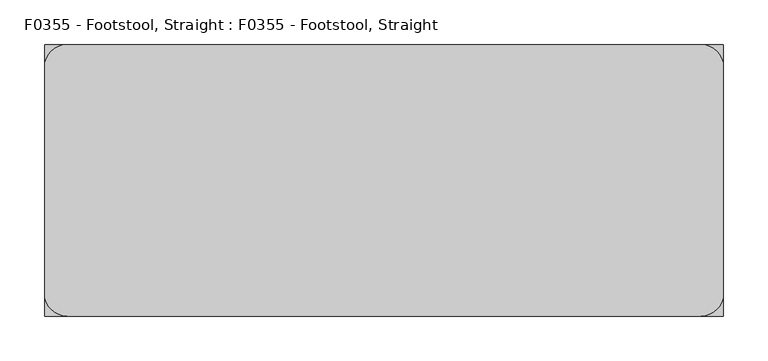
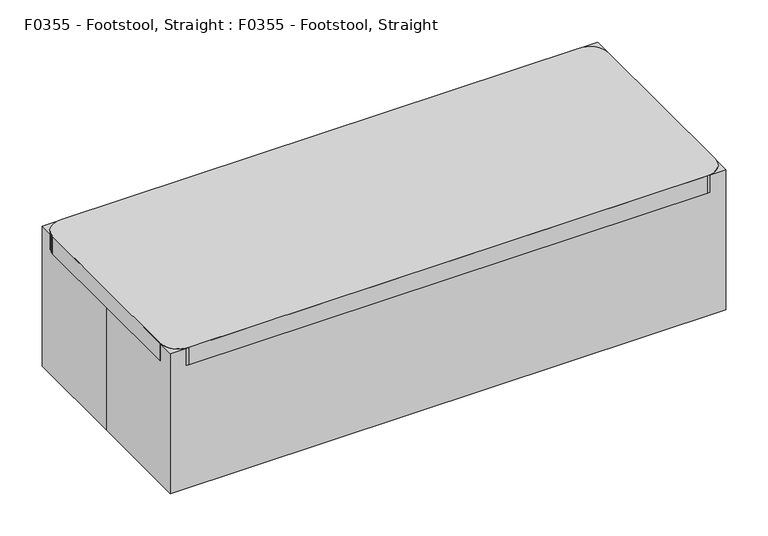
"""IFC4 building model written with IfcOpenShell, lengths in millimetres: proxy geometry, F0355 - Footstool, Straight : F0355 - Footstool, Straight."""

import ifcopenshell
import ifcopenshell.guid

model = None  # the IFC model being written
_history = None  # IfcOwnerHistory: only IFC2X3 demands one
_inside = {}  # id of a spatial element -> (the spatial element, [elements in it])
_under = {}  # id of a project, library or spatial element -> (it, [spatial elements below it])
_declared = {}  # id of a project -> (the project, [libraries it declares])
_typed = {}  # id of a type object -> (the type object, [elements of that type])
_made_of = {}  # id of a material, layer set ... -> (it, [elements and type objects made of it])


def new_model(schema):
    """Start an empty IFC model of exactly this schema.

    Asked for "IFC4X3", IfcOpenShell would pick the latest addendum, in which some entities
    have other attributes; the version numbers below select the first issue.
    IFC2X3 requires an IfcOwnerHistory on every rooted entity: one is made here for all.
    """
    global model, _history
    if schema == "IFC4X3":
        model = ifcopenshell.file(schema_version=(4, 3, 0, 0))
    else:
        model = ifcopenshell.file(schema=schema)
    _inside.clear()
    _under.clear()
    _declared.clear()
    _typed.clear()
    _made_of.clear()
    _history = None
    if model.schema == "IFC2X3":
        org = make("IfcOrganization", Name="unknown")
        user = make(
            "IfcPersonAndOrganization",
            ThePerson=make("IfcPerson", FamilyName="unknown"),
            TheOrganization=org,
        )
        app = make(
            "IfcApplication",
            ApplicationDeveloper=org,
            Version="unknown",
            ApplicationFullName="unknown",
            ApplicationIdentifier="unknown",
        )
        _history = make(
            "IfcOwnerHistory",
            OwningUser=user,
            OwningApplication=app,
            ChangeAction="ADDED",
            CreationDate=0,
        )
    return model


def make(cls, **values):
    """One entity of the class cls with the attributes given. An attribute that is None is left unset."""
    return model.create_entity(
        cls, **{name: value for name, value in values.items() if value is not None}
    )


def rooted(cls, **values):
    """An entity with a GlobalId (a new one), such as an element, a storey or a relation."""
    return make(cls, GlobalId=ifcopenshell.guid.new(), OwnerHistory=_history, **values)


def si_unit(unit_type, name, prefix=None):
    """IfcSIUnit, for example si_unit("LENGTHUNIT", "METRE", prefix="MILLI")."""
    return make("IfcSIUnit", UnitType=unit_type, Prefix=prefix, Name=name)


def assignment(units):
    """IfcUnitAssignment: the units of a project."""
    return None if units is None else make("IfcUnitAssignment", Units=units)


def point(xyz):
    """IfcCartesianPoint."""
    return None if xyz is None else make("IfcCartesianPoint", Coordinates=xyz)


def direction(xyz):
    """IfcDirection."""
    return None if xyz is None else make("IfcDirection", DirectionRatios=xyz)


def frame(location, z_axis=None, x_axis=None):
    """IfcAxis2Placement3D, a coordinate frame: its origin and axes. An axis left out is left unset."""
    return make(
        "IfcAxis2Placement3D",
        Location=point(location),
        Axis=direction(z_axis),
        RefDirection=direction(x_axis),
    )


def frame_2d(location, x_axis=None):
    """IfcAxis2Placement2D, a coordinate frame in the plane: its origin and x axis."""
    return make(
        "IfcAxis2Placement2D", Location=point(location), RefDirection=direction(x_axis)
    )


def origin():
    """The frame at (0, 0, 0) with its axes left unset."""
    return frame((0.0, 0.0, 0.0))


def origin_with_axes():
    """The frame at (0, 0, 0) with the z axis (0, 0, 1) and the x axis (1, 0, 0) written out."""
    return frame((0.0, 0.0, 0.0), z_axis=(0.0, 0.0, 1.0), x_axis=(1.0, 0.0, 0.0))


def place(relative_to, where):
    """IfcLocalPlacement: puts the frame where relative to a parent placement (None: the world)."""
    return make(
        "IfcLocalPlacement", PlacementRelTo=relative_to, RelativePlacement=where
    )


def context(
    kind, dimensions, precision=None, world=None, true_north=None, identifier=None
):
    """IfcGeometricRepresentationContext, for example the 3D "Model" context."""
    return make(
        "IfcGeometricRepresentationContext",
        ContextIdentifier=identifier,
        ContextType=kind,
        CoordinateSpaceDimension=dimensions,
        Precision=precision,
        WorldCoordinateSystem=world,
        TrueNorth=true_north,
    )


def project(units=None, contexts=None):
    """IfcProject with its units and contexts."""
    return rooted(
        "IfcProject",
        Name="project",
        RepresentationContexts=contexts,
        UnitsInContext=assignment(units),
    )


def spatial(cls, under=None, at=None, **own):
    """A site, building, storey or space (cls), placed at a placement, below another one or the project."""
    s = rooted(cls, ObjectPlacement=at, **own)
    if under is not None:
        _under.setdefault(under.id(), (under, []))[1].append(s)
    return s


def polyline(points):
    """IfcPolyline through the points."""
    return make("IfcPolyline", Points=[point(p) for p in points])


def circle_curve(where, radius):
    """IfcCircle in the frame where."""
    return make("IfcCircle", Position=where, Radius=radius)


def trimmed(basis, trim1, trim2, sense, master):
    """IfcTrimmedCurve: the piece of a basis curve between two trims."""
    return make(
        "IfcTrimmedCurve",
        BasisCurve=basis,
        Trim1=trim1,
        Trim2=trim2,
        SenseAgreement=sense,
        MasterRepresentation=master,
    )


def segment(curve, same_sense, transition):
    """IfcCompositeCurveSegment."""
    return make(
        "IfcCompositeCurveSegment",
        Transition=transition,
        SameSense=same_sense,
        ParentCurve=curve,
    )


def composite_curve(segments, self_intersect=None):
    """IfcCompositeCurve: segments joined end to end."""
    return make("IfcCompositeCurve", Segments=segments, SelfIntersect=self_intersect)


def outline(outer, holes=None, kind="AREA"):
    """IfcArbitraryClosedProfileDef: a profile drawn as a closed curve; with holes, ...WithVoids."""
    if holes is None:
        return make("IfcArbitraryClosedProfileDef", ProfileType=kind, OuterCurve=outer)
    return make(
        "IfcArbitraryProfileDefWithVoids",
        ProfileType=kind,
        OuterCurve=outer,
        InnerCurves=holes,
    )


def extrude(swept, where, along, depth):
    """IfcExtrudedAreaSolid: the profile swept, set in the frame where, extruded along a direction by depth."""
    return make(
        "IfcExtrudedAreaSolid",
        SweptArea=swept,
        Position=where,
        ExtrudedDirection=direction(along),
        Depth=depth,
    )


def shape(context_of_items, identifier, shape_type, items):
    """IfcShapeRepresentation: the items that make up one representation, for example the "Body"."""
    return make(
        "IfcShapeRepresentation",
        ContextOfItems=context_of_items,
        RepresentationIdentifier=identifier,
        RepresentationType=shape_type,
        Items=items,
    )


def source(mapping_origin, context_of_items, identifier, shape_type, items):
    """IfcRepresentationMap: a shape defined once, which mapped items show again and again."""
    return make(
        "IfcRepresentationMap",
        MappingOrigin=mapping_origin,
        MappedRepresentation=shape(context_of_items, identifier, shape_type, items),
    )


def transform(
    local_origin,
    x_axis=None,
    y_axis=None,
    z_axis=None,
    scale=None,
    scale2=None,
    scale3=None,
    uniform=True,
):
    """IfcCartesianTransformationOperator3D, or its non-uniform kind. x_axis, y_axis, z_axis: its Axis1, 2, 3."""
    if uniform:
        return make(
            "IfcCartesianTransformationOperator3D",
            Axis1=direction(x_axis),
            Axis2=direction(y_axis),
            LocalOrigin=point(local_origin),
            Scale=scale,
            Axis3=direction(z_axis),
        )
    return make(
        "IfcCartesianTransformationOperator3DnonUniform",
        Axis1=direction(x_axis),
        Axis2=direction(y_axis),
        LocalOrigin=point(local_origin),
        Scale=scale,
        Axis3=direction(z_axis),
        Scale2=scale2,
        Scale3=scale3,
    )


def mapped(mapping_source, mapping_target):
    """IfcMappedItem: shows the shape of a source again, moved by a transform."""
    return make(
        "IfcMappedItem", MappingSource=mapping_source, MappingTarget=mapping_target
    )


def made_of(thing, what):
    """Note that an element or type object is made of a material, layer set ...; save() writes the relation."""
    if what is not None:
        _made_of.setdefault(what.id(), (what, []))[1].append(thing)
    return thing


def element(
    cls,
    number,
    at=None,
    inside=None,
    cuts=None,
    type_object=None,
    material=None,
    context=None,
    identifier="Body",
    shape_type=None,
    held_by="IfcProductDefinitionShape",
    body=None,
    shapes=None,
    **own,
):
    """One element of the class cls, such as IfcWall. Its Tag is "e" and its number.

    at: its placement. inside: the storey or other place that contains it. cuts: it is an
    opening in that element (IfcRelVoidsElement). A single representation is given by context,
    identifier, shape_type and body (its items); several are given by shapes. held_by: the class
    of the entity that holds the representations. save() writes the other relations.
    """
    e = rooted(cls, Tag="e%d" % number, ObjectPlacement=at, **own)
    if body is not None:
        shapes = [shape(context, identifier, shape_type, body)]
    if shapes is not None:
        e.Representation = make(held_by, Representations=shapes)
    if inside is not None:
        _inside.setdefault(inside.id(), (inside, []))[1].append(e)
    if cuts is not None:
        rooted(
            "IfcRelVoidsElement", RelatingBuildingElement=cuts, RelatedOpeningElement=e
        )
    if type_object is not None:
        _typed.setdefault(type_object.id(), (type_object, []))[1].append(e)
    return made_of(e, material)


def aggregate(whole, parts):
    """IfcRelAggregates: a whole, such as a stair, and the parts it consists of."""
    return rooted("IfcRelAggregates", RelatingObject=whole, RelatedObjects=parts)


def save(model, path):
    """Write the relations noted so far, then the file.

    IfcRelAggregates (storeys below a building ...), IfcRelContainedInSpatialStructure (elements
    in a storey), IfcRelDefinesByType, IfcRelAssociatesMaterial and IfcRelDeclares: one each for
    every whole, place, type object, material and project.
    """
    for whole, parts in _under.values():
        aggregate(whole, parts)
    for where, things in _inside.values():
        rooted(
            "IfcRelContainedInSpatialStructure",
            RelatedElements=things,
            RelatingStructure=where,
        )
    for kind, things in _typed.values():
        rooted("IfcRelDefinesByType", RelatedObjects=things, RelatingType=kind)
    for what, things in _made_of.values():
        rooted("IfcRelAssociatesMaterial", RelatedObjects=things, RelatingMaterial=what)
    for by, libraries in _declared.values():
        rooted("IfcRelDeclares", RelatingContext=by, RelatedDefinitions=libraries)
    model.write(path)


def f0355_footstool_straight_f0355_footstool_straight_84fa4ab6(model_context):
    return source(origin(), model_context, "Body", "SweptSolid", [
        extrude(outline(composite_curve([segment(trimmed(circle_curve(frame_2d((-333.6173743, -106.4770511)), 19.05), [point((-352.6673743, -106.4770511))], [point((-314.5673743, -106.4770511))], False, "CARTESIAN"), True, "CONTINUOUS"), segment(trimmed(circle_curve(frame_2d((-333.6173743, -106.4770511)), 19.05), [point((-314.5673743, -106.4770511))], [point((-352.6673743, -106.4770511))], False, "CARTESIAN"), True, "CONTINUOUS")], self_intersect=False)), origin_with_axes(), (0.0, 0.0, 1.0), 177.8),
        extrude(outline(composite_curve([segment(trimmed(circle_curve(frame_2d((-355.6, 127.0)), 25.4), [point((-381.0, 127.0))], [point((-355.6, 152.4))], False, "CARTESIAN"), True, "CONTINUOUS"), segment(polyline([(-355.6, 152.4), (355.6, 152.4)]), True, "CONTINUOUS"), segment(trimmed(circle_curve(frame_2d((355.6, 127.0)), 25.4), [point((355.6, 152.4))], [point((381.0, 127.0))], False, "CARTESIAN"), True, "CONTINUOUS"), segment(polyline([(381.0, 127.0), (381.0, -127.0)]), True, "CONTINUOUS"), segment(trimmed(circle_curve(frame_2d((355.6, -127.0)), 25.4), [point((381.0, -127.0))], [point((355.6, -152.4))], False, "CARTESIAN"), True, "CONTINUOUS"), segment(polyline([(355.6, -152.4), (-355.6, -152.4)]), True, "CONTINUOUS"), segment(trimmed(circle_curve(frame_2d((-355.6, -127.0)), 25.4), [point((-355.6, -152.4))], [point((-381.0, -127.0))], False, "CARTESIAN"), True, "CONTINUOUS"), segment(polyline([(-381.0, -127.0), (-381.0, 127.0)]), True, "CONTINUOUS")], self_intersect=False)), frame((0.0, 0.0, 177.8), z_axis=(0.0, 0.0, 1.0), x_axis=(1.0, 0.0, 0.0)), (0.0, 0.0, 1.0), 25.4),
        extrude(outline(composite_curve([segment(trimmed(circle_curve(frame_2d((333.6173743, 109.4229489)), 19.05), [point((314.5673743, 109.4229489))], [point((352.6673743, 109.4229489))], False, "CARTESIAN"), True, "CONTINUOUS"), segment(trimmed(circle_curve(frame_2d((333.6173743, 109.4229489)), 19.05), [point((352.6673743, 109.4229489))], [point((314.5673743, 109.4229489))], False, "CARTESIAN"), True, "CONTINUOUS")], self_intersect=False)), origin_with_axes(), (0.0, 0.0, 1.0), 177.8),
        extrude(outline(composite_curve([segment(trimmed(circle_curve(frame_2d((-333.6173743, 109.4229489)), 19.05), [point((-352.6673743, 109.4229489))], [point((-314.5673743, 109.4229489))], False, "CARTESIAN"), True, "CONTINUOUS"), segment(trimmed(circle_curve(frame_2d((-333.6173743, 109.4229489)), 19.05), [point((-314.5673743, 109.4229489))], [point((-352.6673743, 109.4229489))], False, "CARTESIAN"), True, "CONTINUOUS")], self_intersect=False)), origin_with_axes(), (0.0, 0.0, 1.0), 177.8),
        extrude(outline(composite_curve([segment(trimmed(circle_curve(frame_2d((333.6173743, -106.4770511)), 19.05), [point((314.5673743, -106.4770511))], [point((352.6673743, -106.4770511))], False, "CARTESIAN"), True, "CONTINUOUS"), segment(trimmed(circle_curve(frame_2d((333.6173743, -106.4770511)), 19.05), [point((352.6673743, -106.4770511))], [point((314.5673743, -106.4770511))], False, "CARTESIAN"), True, "CONTINUOUS")], self_intersect=False)), origin_with_axes(), (0.0, 0.0, 1.0), 177.8),
        extrude(outline(polyline([(-381.0, 152.4), (381.0, 152.4), (381.0, -152.4), (-381.0, -152.4), (-381.0, 0.0), (-381.0, 152.4)])), origin_with_axes(), (0.0, 0.0, 1.0), 203.2),
    ])


if __name__ == "__main__":
    model = new_model("IFC4")
    model_context = context("Model", 3, world=origin())
    ifc_project = project(units=[si_unit("LENGTHUNIT", "METRE", prefix="MILLI")], contexts=[model_context])
    site = spatial("IfcSite", under=ifc_project)
    building = spatial("IfcBuilding", under=site)
    placement = place(None, origin())
    f0355_footstool_straight_f0355_footstool_straight_shape = f0355_footstool_straight_f0355_footstool_straight_84fa4ab6(model_context)
    element("IfcBuildingElementProxy", 1, Name="F0355 - Footstool, Straight : F0355 - Footstool, Straight", ObjectType="F0355 - Footstool, Straight : F0355 - Footstool, Straight", at=placement, inside=building, context=model_context, shape_type="MappedRepresentation", body=[
        mapped(f0355_footstool_straight_f0355_footstool_straight_shape, transform((0.0, 0.0, 0.0), x_axis=(1.0, 0.0, 0.0), y_axis=(0.0, 1.0, 0.0), z_axis=(0.0, 0.0, 1.0))),
    ])
    save(model, "model.ifc")

# Revit data of these elements
# Type "F0355 - Footstool, Straight : F0355 - Footstool, Straight"
#   Watts2 = "0"
#   Watts1 = "0"
#   Unit_Issue = "EA"
#   UTIL_6_Misc = "-"
#   UTIL_5_NonMedGas = "-"
#   UTIL_4_MiscGas = "-"
#   UTIL_3_MedGas = "-"
#   UTIL_2_Elec = "-"
#   UTIL_1_WaterDrain = "-"
#   Nomenclature = "Footstool, Straight"
#   NSN = "6530007086975"
#   Location [instance default] = ""
#   JSN = "F0355"
#   Fund_Source_VA = "-"
#   Fund_Source_Navy = "-"
#   Fund_Source_Army = "-"
#   Fund_Source_AF = "-"
#   ELEC_Volts2 = "0"
#   ELEC_Volts1 = "0"
#   ELEC_Phase2 = "0"
#   ELEC_Phase1 = "0"
#   ELEC_HertzSwitch = "0"
#   ELEC_HertzDependent = "0"
#   ELEC_Hertz = "0"
#   ELEC_Amps2 = "0"
#   ELEC_Amps1 = "0"
#   DetailDescription = "Step stool. Used to assist patients getting on and off exam or surgical tables. Fitted with electrically conductive rubber tips."
#   CAT_VA = "C"
#   CAT_Navy = "C"
#   CAT_IHS = "-"
#   CAT_Army = "C"
#   CAT_AF = "C"
#   BTUperhour = "0"
#   Weight_IP = 19
#   DIM_Width_IP = 2' - 6"
#   DIM_Height_IP = 0' - 8"
#   DIM_Depth_IP = 1' - 0"
# Element 1 (IfcBuildingElementProxy, "F0355 - Footstool, Straight : F0355 - Footstool, Straight")
#   Location = "TRET3"
#   Materials on its faces: "EquipSpace"
# Materials
#   "EquipSpace": class "Unassigned", colour RGB 221 217 195, transparency 0.5
